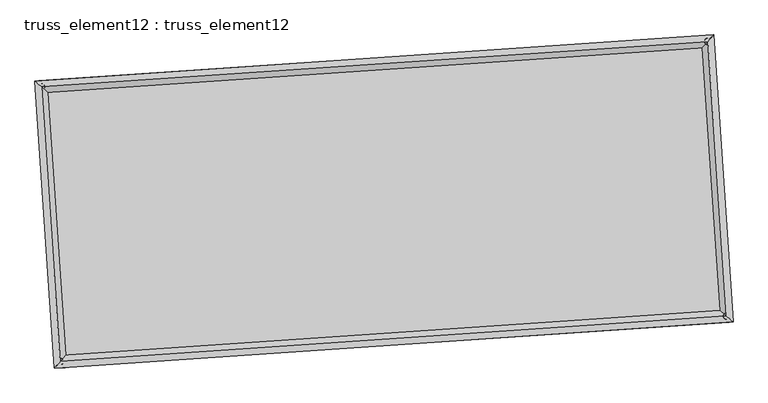
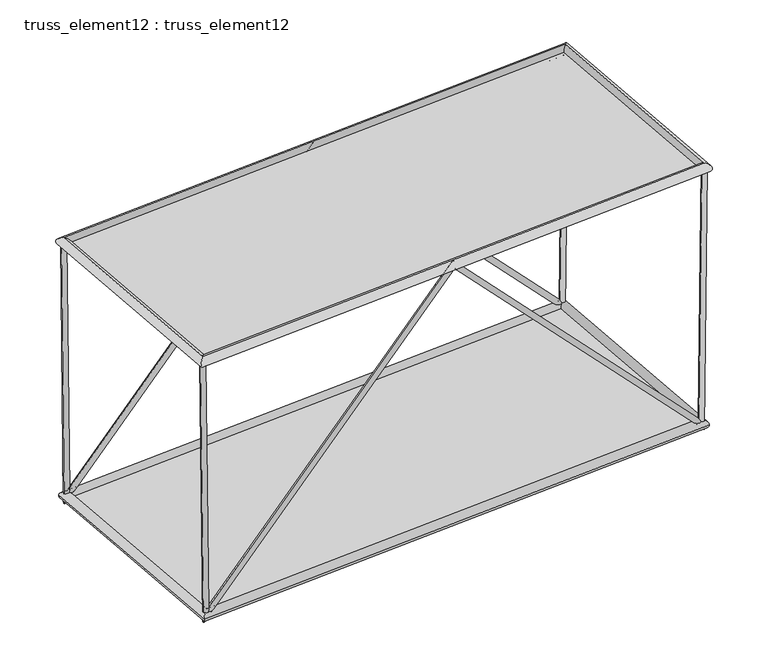
"""IFC4 building model written with IfcOpenShell, lengths in millimetres: plate geometry, truss_element12 : truss_element12."""

from ifc_helpers import new_model, si_unit, frame, origin, origin_with_axes, place, context, project, spatial, polyline, circle_curve, ellipse_curve, outline, extrude, source, transform, mapped, element, save
from ifc_brep_helpers import plane_surface, cylinder_surface, advanced_brep


def truss_element12_truss_element12_752a408a(model_context):
    return source(origin(), model_context, "Body", "SolidModel", [
        advanced_brep(
        [(-3720.8435707, 2272.4122299, 5000.2451385), (-3819.9406863, 2259.0514122, 4999.1270036), (-3666.3111421, 2276.130589, 122.7598556), (-3762.6757407, 2262.9560911, -122.7598556), (1064.2284648, 2598.6881023, 5071.8018968), (1064.6690654, 2592.114383, 4927.5587925), (5793.7746069, 2921.177875, 122.752757), (5890.9863701, 2921.2026135, -122.752757), (5849.2930132, 2924.9634641, 5000.243792), (5949.286304, 2925.1778643, 4999.1054445)],
        [
            (0, 1, circle_curve(frame((-3770.3921285, 2265.7318211, 4999.6860711), z_axis=(-0.011179737411859392, -0.0007623037959541654, 0.9999372142111348), x_axis=(-0.13360831246989213, 0.9910339417884559, -0.0007382832674076436)), 50.0)),
            (1, 0, circle_curve(frame((-3770.3921285, 2265.7318211, 4999.6860711), z_axis=(-0.011179737411859392, -0.0007623037959541654, 0.9999372142111348), x_axis=(-0.13360831246989213, 0.9910339417884559, -0.0007382832674076436)), 50.0)),
            (0, 2),
            (2, 3, ellipse_curve(frame((-3714.4934414, 2269.54334, 0.0), z_axis=(-0.9278429760300566, -0.06326608547413519, 0.36756606788503654), x_axis=(0.3667145628894319, 0.025004872030869717, 0.9299974116843192)), 132.2876405, 50.0)),
            (3, 1),
            (3, 2, ellipse_curve(frame((-3714.4934414, 2269.54334, 0.0), z_axis=(-0.9278429760300566, -0.06326608547413519, 0.36756606788503654), x_axis=(0.3667145628894319, 0.025004872030869717, 0.9299974116843192)), 132.2876405, 50.0)),
            (2, 4),
            (4, 5, ellipse_curve(frame((1064.4487651, 2595.4012426, 4999.6803447), z_axis=(-0.9976833946832315, -0.06802823813380893, 5.28181136524599e-05), x_axis=(-5.269575500290447e-05, -3.593123218295458e-06, -0.9999999986051235)), 72.2785958, 50.0)),
            (5, 3),
            (5, 4, ellipse_curve(frame((1064.4487651, 2595.4012426, 4999.6803447), z_axis=(-0.9976833946832315, -0.06802823813380893, 5.28181136524599e-05), x_axis=(-5.269575500290447e-05, -3.593123218295458e-06, -0.9999999986051235)), 72.2785958, 50.0)),
            (4, 6),
            (6, 7, ellipse_curve(frame((5842.3804885, 2921.1902443, 0.0), z_axis=(-0.9278994784854568, -0.06326993816178289, -0.36742274392234003), x_axis=(-0.3665715709515899, -0.024995121954191606, 0.9300540453374624)), 132.271936, 50.0)),
            (7, 5),
            (7, 6, ellipse_curve(frame((5842.3804885, 2921.1902443, 0.0), z_axis=(-0.9278994784854568, -0.06326993816178289, -0.36742274392234003), x_axis=(-0.3665715709515899, -0.024995121954191606, 0.9300540453374624)), 132.271936, 50.0)),
            (8, 9, circle_curve(frame((5899.2896586, 2925.0706642, 4999.6746183), z_axis=(0.011381834017518641, 0.000776083995252831, 0.9999349236565498), x_axis=(-0.0021526974028054716, 0.9999974004703052, -0.0007516292465537602)), 50.0)),
            (9, 8, circle_curve(frame((5899.2896586, 2925.0706642, 4999.6746183), z_axis=(0.011381834017518641, 0.000776083995252831, 0.9999349236565498), x_axis=(-0.0021526974028054716, 0.9999974004703052, -0.0007516292465537602)), 50.0)),
            (6, 8),
            (9, 7),
        ],
        [
            plane_surface(frame((-3770.3921285, 2315.7318065, 4999.7241886), z_axis=(-0.011179737411861788, -0.0007623037959489812, 0.9999372142111346), x_axis=(0.9999375047828748, -8.522888906625786e-06, 0.011179734163143003))),
            cylinder_surface(frame((-3770.3921285, 2265.7318211, 4999.6860711), z_axis=(-0.011179737411859392, -0.0007623037959541654, 0.9999372142111348), x_axis=(-0.13360831246989213, 0.9910339417884559, -0.0007382832674076436)), 50.0),
            cylinder_surface(frame((-3714.4934414, 2269.54334, 0.0), z_axis=(-0.6902032279648624, -0.04706233440682364, -0.7220835414182107), x_axis=(-0.020416427197213927, 0.9987520661625611, -0.045579379509995036)), 50.0),
            cylinder_surface(frame((1064.4487651, 2595.4012426, 4999.6803447), z_axis=(-0.690127122639195, -0.047057145073969846, 0.7221566171511784), x_axis=(-0.1153492355275266, 0.9922789588359066, -0.045574353695306324)), 50.0),
            plane_surface(frame((5899.2896586, 2875.0706793, 4999.713425), z_axis=(0.01138183401752019, 0.0007760839952526793, 0.9999349236565498), x_axis=(0.9999352248292875, -8.833831429910796e-06, -0.011381830589400023))),
            cylinder_surface(frame((5842.3804885, 2921.1902443, 0.0), z_axis=(-0.011381834017518641, -0.000776083995252831, -0.9999349236565498), x_axis=(-0.0021526974028054716, 0.9999974004703052, -0.0007516292465537602)), 50.0),
        ],
        [
            (0, [[1, 2]]),
            (1, [[-1, 3, 4, 5]]),
            (1, [[-2, -5, 6, -3]]),
            (2, [[-4, 7, 8, 9]]),
            (2, [[-6, -9, 10, -7]]),
            (3, [[-8, 11, 12, 13]]),
            (3, [[-10, -13, 14, -11]]),
            (4, [[15, 16]]),
            (5, [[-12, 17, -16, 18]]),
            (5, [[-14, -18, -15, -17]]),
        ],
    ),
        advanced_brep(
        [(-3448.7306178, -1718.3213544, 5000.2451385), (-3547.8277334, -1731.6821721, 4999.1270036), (-3394.1981892, -1714.6029953, 122.7598556), (-3490.5627878, -1727.7774932, -122.7598556), (1336.3414177, -1392.045482, 5071.8018968), (1336.7820183, -1398.6192013, 4927.5587925), (6065.8875598, -1069.5557093, 122.752757), (6163.099323, -1069.5309708, -122.752757), (6121.4059661, -1065.7701202, 5000.243792), (6221.3992569, -1065.55572, 4999.1054445)],
        [
            (0, 1, circle_curve(frame((-3498.2791756, -1725.0017632, 4999.6860711), z_axis=(-0.01117973741185968, -0.0007623037959541836, 0.9999372142111347), x_axis=(-0.1336083124698922, 0.9910339417884559, -0.0007382832674076648)), 50.0)),
            (1, 0, circle_curve(frame((-3498.2791756, -1725.0017632, 4999.6860711), z_axis=(-0.01117973741185968, -0.0007623037959541836, 0.9999372142111347), x_axis=(-0.1336083124698922, 0.9910339417884559, -0.0007382832674076648)), 50.0)),
            (0, 2),
            (2, 3, ellipse_curve(frame((-3442.3804885, -1721.1902443, 0.0), z_axis=(-0.9278429760300567, -0.06326608547413527, 0.36756606788503626), x_axis=(0.3667145628894316, 0.025004872030869728, 0.9299974116843192)), 132.2876405, 50.0)),
            (3, 1),
            (3, 2, ellipse_curve(frame((-3442.3804885, -1721.1902443, 0.0), z_axis=(-0.9278429760300567, -0.06326608547413527, 0.36756606788503626), x_axis=(0.3667145628894316, 0.025004872030869728, 0.9299974116843192)), 132.2876405, 50.0)),
            (2, 4),
            (4, 5, ellipse_curve(frame((1336.561718, -1395.3323417, 4999.6803447), z_axis=(-0.9976833946832315, -0.06802823813380908, 5.281811365229941e-05), x_axis=(-5.269575500275073e-05, -3.593123218208977e-06, -0.9999999986051235)), 72.2785958, 50.0)),
            (5, 3),
            (5, 4, ellipse_curve(frame((1336.561718, -1395.3323417, 4999.6803447), z_axis=(-0.9976833946832315, -0.06802823813380908, 5.281811365229941e-05), x_axis=(-5.269575500275073e-05, -3.593123218208977e-06, -0.9999999986051235)), 72.2785958, 50.0)),
            (4, 6),
            (6, 7, ellipse_curve(frame((6114.4934414, -1069.54334, 0.0), z_axis=(-0.9278994784854566, -0.0632699381617831, -0.36742274392234037), x_axis=(-0.36657157095159015, -0.024995121954191686, 0.9300540453374623)), 132.271936, 50.0)),
            (7, 5),
            (7, 6, ellipse_curve(frame((6114.4934414, -1069.54334, 0.0), z_axis=(-0.9278994784854566, -0.0632699381617831, -0.36742274392234037), x_axis=(-0.36657157095159015, -0.024995121954191686, 0.9300540453374623)), 132.271936, 50.0)),
            (8, 9, circle_curve(frame((6171.4026115, -1065.6629201, 4999.6746183), z_axis=(0.011381834017518487, 0.0007760839952528411, 0.9999349236565498), x_axis=(-0.0021526974028057495, 0.999997400470305, -0.0007516292465537674)), 50.0)),
            (9, 8, circle_curve(frame((6171.4026115, -1065.6629201, 4999.6746183), z_axis=(0.011381834017518487, 0.0007760839952528411, 0.9999349236565498), x_axis=(-0.0021526974028057495, 0.999997400470305, -0.0007516292465537674)), 50.0)),
            (6, 8),
            (9, 7),
        ],
        [
            plane_surface(frame((-3498.2791756, -1675.0017778, 4999.7241886), z_axis=(-0.011179737411861788, -0.0007623037959489832, 0.9999372142111346), x_axis=(0.9999375047828748, -8.522888906625786e-06, 0.011179734163143003))),
            cylinder_surface(frame((-3498.2791756, -1725.0017632, 4999.6860711), z_axis=(-0.01117973741185968, -0.0007623037959541836, 0.9999372142111347), x_axis=(-0.1336083124698922, 0.9910339417884559, -0.0007382832674076648)), 50.0),
            cylinder_surface(frame((-3442.3804885, -1721.1902443, 0.0), z_axis=(-0.6902032279648624, -0.04706233440682368, -0.7220835414182106), x_axis=(-0.020416427197213982, 0.9987520661625612, -0.04557937950999504)), 50.0),
            cylinder_surface(frame((1336.561718, -1395.3323417, 4999.6803447), z_axis=(-0.690127122639195, -0.047057145073969985, 0.7221566171511782), x_axis=(-0.11534923552752677, 0.9922789588359064, -0.04557435369530631)), 50.0),
            plane_surface(frame((6171.4026115, -1115.662905, 4999.713425), z_axis=(0.01138183401752019, 0.0007760839952526833, 0.9999349236565498), x_axis=(0.9999352248292875, -8.833831430354886e-06, -0.011381830589400023))),
            cylinder_surface(frame((6114.4934414, -1069.54334, 0.0), z_axis=(-0.011381834017518487, -0.0007760839952528411, -0.9999349236565498), x_axis=(-0.0021526974028057495, 0.999997400470305, -0.0007516292465537674)), 50.0),
        ],
        [
            (0, [[1, 2]]),
            (1, [[-1, 3, 4, 5]]),
            (1, [[-2, -5, 6, -3]]),
            (2, [[-4, 7, 8, 9]]),
            (2, [[-6, -9, 10, -7]]),
            (3, [[-8, 11, 12, 13]]),
            (3, [[-10, -13, 14, -11]]),
            (4, [[15, 16]]),
            (5, [[-12, 17, -16, 18]]),
            (5, [[-14, -18, -15, -17]]),
        ],
    ),
        advanced_brep(
        [(-3498.282185, -1725.0050987, 4909.6860711), (-3498.2761662, -1724.9984278, 5089.686071), (-3770.3886942, 2265.728925, 5089.686071), (-3770.3955628, 2265.7347171, 4909.6860711), (5899.2868614, 2925.0673433, 5089.6746182), (5899.2924558, 2925.0739852, 4909.6746183), (6171.3993894, -1065.6600095, 5089.6746182), (6171.4058336, -1065.6658306, 4909.6746183)],
        [
            (0, 1, ellipse_curve(frame((-3498.2791756, -1725.0017632, 4999.6860711), z_axis=(-0.7535719234049665, 0.6573654662781132, 8.355572552120736e-07), x_axis=(-0.6573654662775871, -0.7535719234054254, 8.35557255212046e-07)), 127.2792206, 90.0)),
            (1, 2),
            (2, 3, ellipse_curve(frame((-3770.3921285, 2265.7318211, 4999.6860711), z_axis=(-0.6573654662775872, -0.7535719234054254, 8.355572552120183e-07), x_axis=(0.7535719234049666, -0.6573654662781131, -8.355572552120459e-07)), 127.2792206, 90.0)),
            (3, 0),
            (1, 0, ellipse_curve(frame((-3498.2791756, -1725.0017632, 4999.6860711), z_axis=(-0.7535719234049665, 0.6573654662781132, 8.355572552120736e-07), x_axis=(-0.6573654662775871, -0.7535719234054254, 8.35557255212046e-07)), 127.2792206, 90.0)),
            (3, 2, ellipse_curve(frame((-3770.3921285, 2265.7318211, 4999.6860711), z_axis=(-0.6573654662775872, -0.7535719234054254, 8.355572552120183e-07), x_axis=(0.7535719234049666, -0.6573654662781131, -8.355572552120459e-07)), 127.2792206, 90.0)),
            (2, 4),
            (4, 5, ellipse_curve(frame((5899.2896586, 2925.0706642, 4999.6746183), z_axis=(-0.7535719234049664, 0.6573654662781134, 8.355572552120178e-07), x_axis=(-0.6573654662775871, -0.7535719234054254, 8.355572552120462e-07)), 127.2792206, 90.0)),
            (5, 3),
            (5, 4, ellipse_curve(frame((5899.2896586, 2925.0706642, 4999.6746183), z_axis=(-0.7535719234049664, 0.6573654662781134, 8.355572552120178e-07), x_axis=(-0.6573654662775871, -0.7535719234054254, 8.355572552120462e-07)), 127.2792206, 90.0)),
            (4, 6),
            (6, 7, ellipse_curve(frame((6171.4026115, -1065.6629201, 4999.6746183), z_axis=(0.6573654662775874, 0.7535719234054251, -8.355572552120743e-07), x_axis=(-0.7535719234049663, 0.6573654662781134, 8.355572552120455e-07)), 127.2792206, 90.0)),
            (7, 5),
            (7, 6, ellipse_curve(frame((6171.4026115, -1065.6629201, 4999.6746183), z_axis=(0.6573654662775874, 0.7535719234054251, -8.355572552120743e-07), x_axis=(-0.7535719234049663, 0.6573654662781134, 8.355572552120455e-07)), 127.2792206, 90.0)),
            (6, 1),
            (0, 7),
        ],
        [
            cylinder_surface(frame((-3498.2791756, -1725.0017632, 4999.6860711), z_axis=(0.06802823822870423, -0.9976833960748764, 0.0), x_axis=(-0.9976833954326235, -0.06802823818491144, 3.588159036759498e-05)), 90.0),
            cylinder_surface(frame((-3770.3921285, 2265.7318211, 4999.6860711), z_axis=(-0.9976833960741801, -0.06802823822865382, 1.1816564024600931e-06), x_axis=(-0.06802823814683699, 0.997683395477018, 3.469993396584626e-05)), 90.0),
            cylinder_surface(frame((5899.2896586, 2925.0706642, 4999.6746183), z_axis=(-0.06802823822870385, 0.9976833960748764, 0.0), x_axis=(0.9976833955144403, 0.06802823819048984, 3.3518277564097554e-05)), 90.0),
            cylinder_surface(frame((6171.4026115, -1065.6629201, 4999.6746183), z_axis=(0.99768339607418, 0.06802823822865364, -1.1816564024601325e-06), x_axis=(0.06802823822865364, -0.9976833954714391, 3.469993396584625e-05)), 90.0),
        ],
        [
            (0, [[1, 2, 3, 4]]),
            (0, [[5, -4, 6, -2]]),
            (1, [[-3, 7, 8, 9]]),
            (1, [[-6, -9, 10, -7]]),
            (2, [[-8, 11, 12, 13]]),
            (2, [[-10, -13, 14, -11]]),
            (3, [[-12, 15, -1, 16]]),
            (3, [[-14, -16, -5, -15]]),
        ],
    ),
        advanced_brep(
        [(-3358.7115243, -1625.2761972, 0.0), (-3526.0494527, -1817.1042913, 0.0), (-3810.4074885, 2353.2123043, 0.0), (-3618.5793943, 2185.8743758, 0.0), (5926.0494527, 3017.1042913, 0.0), (5758.7115243, 2825.2761972, 0.0), (6210.4074885, -1153.2123043, 0.0), (6018.5793943, -985.8743758, 0.0)],
        [
            (0, 1, ellipse_curve(frame((-3442.3804885, -1721.1902443, 0.0), z_axis=(-0.7535719234054584, 0.6573654662780803, 0.0), x_axis=(-0.6573654662780803, -0.7535719234054582, 0.0)), 127.2792206, 90.0)),
            (1, 2),
            (2, 3, ellipse_curve(frame((-3714.4934414, 2269.54334, 0.0), z_axis=(-0.6573654662780803, -0.7535719234054584, 0.0), x_axis=(0.7535719234054585, -0.6573654662780801, 0.0)), 127.2792206, 90.0)),
            (3, 0),
            (1, 0, ellipse_curve(frame((-3442.3804885, -1721.1902443, 0.0), z_axis=(-0.7535719234054584, 0.6573654662780803, 0.0), x_axis=(-0.6573654662780803, -0.7535719234054582, 0.0)), 127.2792206, 90.0)),
            (3, 2, ellipse_curve(frame((-3714.4934414, 2269.54334, 0.0), z_axis=(-0.6573654662780803, -0.7535719234054584, 0.0), x_axis=(0.7535719234054585, -0.6573654662780801, 0.0)), 127.2792206, 90.0)),
            (2, 4),
            (4, 5, ellipse_curve(frame((5842.3804885, 2921.1902443, 0.0), z_axis=(-0.7535719234054583, 0.6573654662780805, 0.0), x_axis=(-0.6573654662780805, -0.7535719234054583, 0.0)), 127.2792206, 90.0)),
            (5, 3),
            (5, 4, ellipse_curve(frame((5842.3804885, 2921.1902443, 0.0), z_axis=(-0.7535719234054583, 0.6573654662780805, 0.0), x_axis=(-0.6573654662780805, -0.7535719234054583, 0.0)), 127.2792206, 90.0)),
            (4, 6),
            (6, 7, ellipse_curve(frame((6114.4934414, -1069.54334, 0.0), z_axis=(0.6573654662780806, 0.7535719234054582, 0.0), x_axis=(-0.7535719234054582, 0.6573654662780805, 0.0)), 127.2792206, 90.0)),
            (7, 5),
            (7, 6, ellipse_curve(frame((6114.4934414, -1069.54334, 0.0), z_axis=(0.6573654662780806, 0.7535719234054582, 0.0), x_axis=(-0.7535719234054582, 0.6573654662780805, 0.0)), 127.2792206, 90.0)),
            (6, 1),
            (0, 7),
        ],
        [
            cylinder_surface(frame((-3442.3804885, -1721.1902443, 0.0), z_axis=(0.06802823822870338, -0.9976833960748764, 0.0), x_axis=(-0.9976833960748764, -0.06802823822870338, 0.0)), 90.0),
            cylinder_surface(frame((-3714.4934414, 2269.54334, 0.0), z_axis=(-0.9976833960748767, -0.06802823822870045, 0.0), x_axis=(-0.06802823822870045, 0.9976833960748767, 0.0)), 90.0),
            cylinder_surface(frame((5842.3804885, 2921.1902443, 0.0), z_axis=(-0.06802823822870308, 0.9976833960748764, 0.0), x_axis=(0.9976833960748764, 0.06802823822870308, 0.0)), 90.0),
            cylinder_surface(frame((6114.4934414, -1069.54334, 0.0), z_axis=(0.9976833960748768, 0.06802823822870013, 0.0), x_axis=(0.06802823822870013, -0.9976833960748768, 0.0)), 90.0),
        ],
        [
            (0, [[1, 2, 3, 4]]),
            (0, [[5, -4, 6, -2]]),
            (1, [[-3, 7, 8, 9]]),
            (1, [[-6, -9, 10, -7]]),
            (2, [[-8, 11, 12, 13]]),
            (2, [[-10, -13, 14, -11]]),
            (3, [[-12, 15, -1, 16]]),
            (3, [[-14, -16, -5, -15]]),
        ],
    ),
        extrude(outline(polyline([(-3442.3804885, -1721.1902443), (-3714.4934414, 2269.54334), (5842.3804885, 2921.1902443), (6114.4934414, -1069.54334), (-3442.3804885, -1721.1902443)])), origin_with_axes(), (0.0, 0.0, 1.0), 20.0),
        extrude(outline(polyline([(-2000.0, 4846.0673121), (2000.0, 4846.0673121), (2000.0, -4846.0673121), (-2000.0, -4846.0673121), (-2000.0, 4846.0673121)])), frame((1200.5052415, 600.0344505, 4999.6803447), z_axis=(1.1789189726000265e-06, 8.038600325102859e-08, 0.9999999999993019), x_axis=(-0.0680282382287029, 0.9976833960748765, 0.0)), (0.0, 0.0, 1.0), 20.0),
    ])


if __name__ == "__main__":
    model = new_model("IFC4")
    model_context = context("Model", 3, world=origin())
    ifc_project = project(units=[si_unit("LENGTHUNIT", "METRE", prefix="MILLI")], contexts=[model_context])
    site = spatial("IfcSite", under=ifc_project)
    building = spatial("IfcBuilding", under=site)
    placement = place(None, origin())
    truss_element12_truss_element12_shape = truss_element12_truss_element12_752a408a(model_context)
    element("IfcPlate", 1, ObjectType="truss_element12 : truss_element12", at=placement, inside=building, context=model_context, shape_type="MappedRepresentation", body=[
        mapped(truss_element12_truss_element12_shape, transform((0.0, 0.0, 0.0), x_axis=(1.0, 0.0, 0.0), y_axis=(0.0, 1.0, 0.0), z_axis=(0.0, 0.0, 1.0))),
    ])
    save(model, "model.ifc")

# Revit data of these elements
# Type "truss_element12 : truss_element12"
#   steellbar1 = 90 mm
#   steelbar2 = 50 mm
#   offset1 = 5000 mm
#   M = Default Roof
# Element 1 (IfcPlate, "truss_element12 : truss_element12")
#   Materials on its faces: "Default Roof"
# Materials
#   "Default Roof": class "Miscellaneous", colour RGB 0 127 0, transparency 0, Comments = "Rendering appearance not upgraded Rendering appearance not upgraded ", Cost = 0
